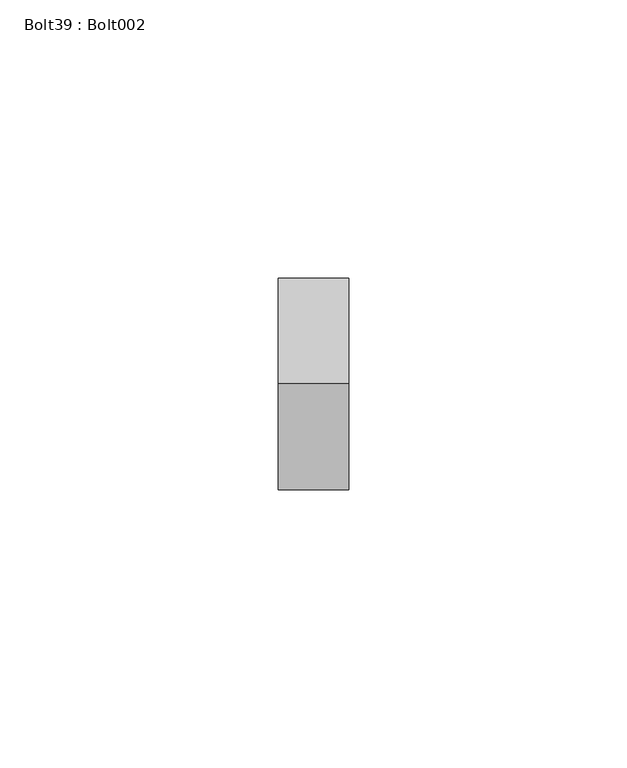
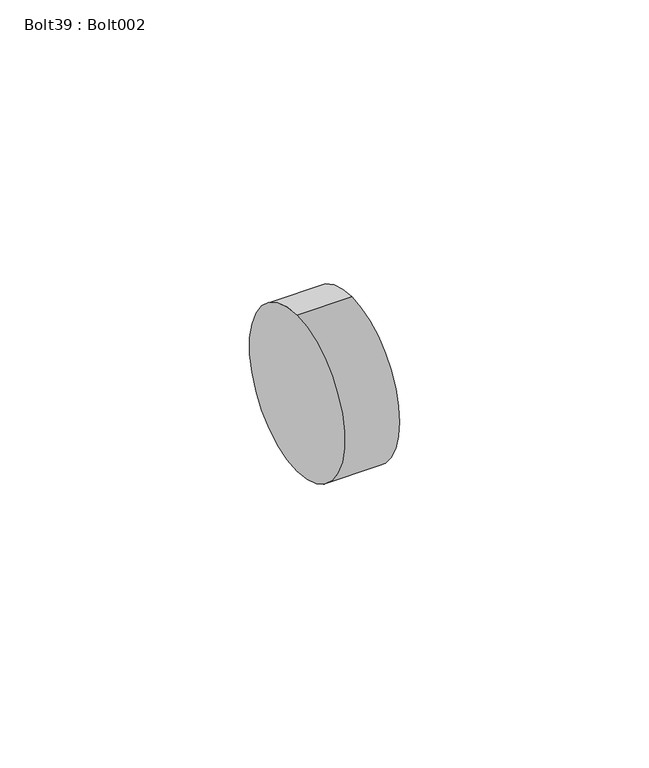
"""IFC4 building model written with IfcOpenShell, lengths in millimetres: proxy geometry, Bolt39 : Bolt002."""

from ifc_helpers import new_model, si_unit, point, frame, frame_2d, origin, place, context, project, spatial, circle_curve, trimmed, segment, composite_curve, outline, extrude, source, transform, mapped, element, save


def bolt39_bolt002_8e1fe756(model_context):
    return source(origin(), model_context, "Body", "SweptSolid", [
        extrude(outline(composite_curve([segment(trimmed(circle_curve(frame_2d((1985.8304801, 39960.0063132)), 19.05), [point((1985.8304801, 39979.0563132))], [point((1985.8304801, 39940.9563132))], False, "CARTESIAN"), True, "CONTINUOUS"), segment(trimmed(circle_curve(frame_2d((1985.8304801, 39960.0063132)), 19.05), [point((1985.8304801, 39940.9563132))], [point((1985.8304801, 39979.0563132))], False, "CARTESIAN"), True, "CONTINUOUS")], self_intersect=False)), frame((10268.2640809, 0.0, 0.0), z_axis=(1.0, 0.0, 0.0), x_axis=(0.0, 1.0, 0.0)), (0.0, 0.0, 1.0), 12.7),
    ])


if __name__ == "__main__":
    model = new_model("IFC4")
    model_context = context("Model", 3, world=origin())
    ifc_project = project(units=[si_unit("LENGTHUNIT", "METRE", prefix="MILLI")], contexts=[model_context])
    site = spatial("IfcSite", under=ifc_project)
    building = spatial("IfcBuilding", under=site)
    placement = place(None, origin())
    bolt39_bolt002_shape = bolt39_bolt002_8e1fe756(model_context)
    element("IfcBuildingElementProxy", 1, Name="Bolt39 : Bolt002", ObjectType="Bolt39 : Bolt002", at=placement, inside=building, context=model_context, shape_type="MappedRepresentation", body=[
        mapped(bolt39_bolt002_shape, transform((0.0, 0.0, 0.0), x_axis=(1.0, 0.0, 0.0), y_axis=(0.0, 1.0, 0.0), z_axis=(0.0, 0.0, 1.0))),
    ])
    save(model, "model.ifc")

# Revit data of these elements
# Type "Bolt39 : Bolt002"
#   NameOverride = "Bolt002"
# Element 1 (IfcBuildingElementProxy, "Bolt39 : Bolt002")
#   Materials on its faces: "STEEL ANGLE AND ANCHOR BOLT (SEE STRUCT. DWGS)"
# Materials
#   "STEEL ANGLE AND ANCHOR BOLT (SEE STRUCT. DWGS)": class "Unassigned", colour RGB 128 128 128, transparency 0, Cost = 0
